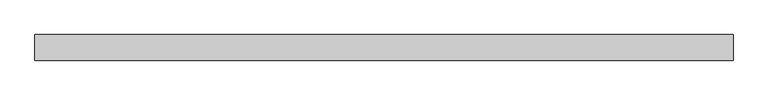
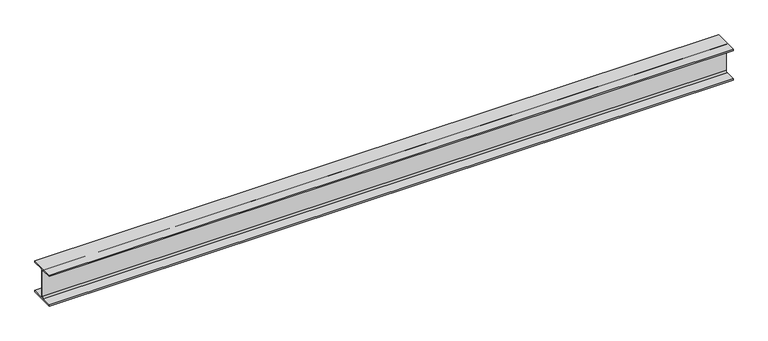
"""IFC4 building model written with IfcOpenShell, lengths in millimetres: beam geometry, 0912_Steel Framing_H-KSD3502 : H_SB_ASB_H-390x300x10x16."""

import ifcopenshell
import ifcopenshell.guid

model = None  # the IFC model being written
_history = None  # IfcOwnerHistory: only IFC2X3 demands one
_inside = {}  # id of a spatial element -> (the spatial element, [elements in it])
_under = {}  # id of a project, library or spatial element -> (it, [spatial elements below it])
_declared = {}  # id of a project -> (the project, [libraries it declares])
_typed = {}  # id of a type object -> (the type object, [elements of that type])
_made_of = {}  # id of a material, layer set ... -> (it, [elements and type objects made of it])


def new_model(schema):
    """Start an empty IFC model of exactly this schema.

    Asked for "IFC4X3", IfcOpenShell would pick the latest addendum, in which some entities
    have other attributes; the version numbers below select the first issue.
    IFC2X3 requires an IfcOwnerHistory on every rooted entity: one is made here for all.
    """
    global model, _history
    if schema == "IFC4X3":
        model = ifcopenshell.file(schema_version=(4, 3, 0, 0))
    else:
        model = ifcopenshell.file(schema=schema)
    _inside.clear()
    _under.clear()
    _declared.clear()
    _typed.clear()
    _made_of.clear()
    _history = None
    if model.schema == "IFC2X3":
        org = make("IfcOrganization", Name="unknown")
        user = make(
            "IfcPersonAndOrganization",
            ThePerson=make("IfcPerson", FamilyName="unknown"),
            TheOrganization=org,
        )
        app = make(
            "IfcApplication",
            ApplicationDeveloper=org,
            Version="unknown",
            ApplicationFullName="unknown",
            ApplicationIdentifier="unknown",
        )
        _history = make(
            "IfcOwnerHistory",
            OwningUser=user,
            OwningApplication=app,
            ChangeAction="ADDED",
            CreationDate=0,
        )
    return model


def make(cls, **values):
    """One entity of the class cls with the attributes given. An attribute that is None is left unset."""
    return model.create_entity(
        cls, **{name: value for name, value in values.items() if value is not None}
    )


def rooted(cls, **values):
    """An entity with a GlobalId (a new one), such as an element, a storey or a relation."""
    return make(cls, GlobalId=ifcopenshell.guid.new(), OwnerHistory=_history, **values)


def si_unit(unit_type, name, prefix=None):
    """IfcSIUnit, for example si_unit("LENGTHUNIT", "METRE", prefix="MILLI")."""
    return make("IfcSIUnit", UnitType=unit_type, Prefix=prefix, Name=name)


def assignment(units):
    """IfcUnitAssignment: the units of a project."""
    return None if units is None else make("IfcUnitAssignment", Units=units)


def point(xyz):
    """IfcCartesianPoint."""
    return None if xyz is None else make("IfcCartesianPoint", Coordinates=xyz)


def direction(xyz):
    """IfcDirection."""
    return None if xyz is None else make("IfcDirection", DirectionRatios=xyz)


def frame(location, z_axis=None, x_axis=None):
    """IfcAxis2Placement3D, a coordinate frame: its origin and axes. An axis left out is left unset."""
    return make(
        "IfcAxis2Placement3D",
        Location=point(location),
        Axis=direction(z_axis),
        RefDirection=direction(x_axis),
    )


def frame_2d(location, x_axis=None):
    """IfcAxis2Placement2D, a coordinate frame in the plane: its origin and x axis."""
    return make(
        "IfcAxis2Placement2D", Location=point(location), RefDirection=direction(x_axis)
    )


def origin():
    """The frame at (0, 0, 0) with its axes left unset."""
    return frame((0.0, 0.0, 0.0))


def place(relative_to, where):
    """IfcLocalPlacement: puts the frame where relative to a parent placement (None: the world)."""
    return make(
        "IfcLocalPlacement", PlacementRelTo=relative_to, RelativePlacement=where
    )


def context(
    kind, dimensions, precision=None, world=None, true_north=None, identifier=None
):
    """IfcGeometricRepresentationContext, for example the 3D "Model" context."""
    return make(
        "IfcGeometricRepresentationContext",
        ContextIdentifier=identifier,
        ContextType=kind,
        CoordinateSpaceDimension=dimensions,
        Precision=precision,
        WorldCoordinateSystem=world,
        TrueNorth=true_north,
    )


def project(units=None, contexts=None):
    """IfcProject with its units and contexts."""
    return rooted(
        "IfcProject",
        Name="project",
        RepresentationContexts=contexts,
        UnitsInContext=assignment(units),
    )


def spatial(cls, under=None, at=None, **own):
    """A site, building, storey or space (cls), placed at a placement, below another one or the project."""
    s = rooted(cls, ObjectPlacement=at, **own)
    if under is not None:
        _under.setdefault(under.id(), (under, []))[1].append(s)
    return s


def polyline(points):
    """IfcPolyline through the points."""
    return make("IfcPolyline", Points=[point(p) for p in points])


def circle_curve(where, radius):
    """IfcCircle in the frame where."""
    return make("IfcCircle", Position=where, Radius=radius)


def trimmed(basis, trim1, trim2, sense, master):
    """IfcTrimmedCurve: the piece of a basis curve between two trims."""
    return make(
        "IfcTrimmedCurve",
        BasisCurve=basis,
        Trim1=trim1,
        Trim2=trim2,
        SenseAgreement=sense,
        MasterRepresentation=master,
    )


def segment(curve, same_sense, transition):
    """IfcCompositeCurveSegment."""
    return make(
        "IfcCompositeCurveSegment",
        Transition=transition,
        SameSense=same_sense,
        ParentCurve=curve,
    )


def composite_curve(segments, self_intersect=None):
    """IfcCompositeCurve: segments joined end to end."""
    return make("IfcCompositeCurve", Segments=segments, SelfIntersect=self_intersect)


def outline(outer, holes=None, kind="AREA"):
    """IfcArbitraryClosedProfileDef: a profile drawn as a closed curve; with holes, ...WithVoids."""
    if holes is None:
        return make("IfcArbitraryClosedProfileDef", ProfileType=kind, OuterCurve=outer)
    return make(
        "IfcArbitraryProfileDefWithVoids",
        ProfileType=kind,
        OuterCurve=outer,
        InnerCurves=holes,
    )


def extrude(swept, where, along, depth):
    """IfcExtrudedAreaSolid: the profile swept, set in the frame where, extruded along a direction by depth."""
    return make(
        "IfcExtrudedAreaSolid",
        SweptArea=swept,
        Position=where,
        ExtrudedDirection=direction(along),
        Depth=depth,
    )


def shape(context_of_items, identifier, shape_type, items):
    """IfcShapeRepresentation: the items that make up one representation, for example the "Body"."""
    return make(
        "IfcShapeRepresentation",
        ContextOfItems=context_of_items,
        RepresentationIdentifier=identifier,
        RepresentationType=shape_type,
        Items=items,
    )


def source(mapping_origin, context_of_items, identifier, shape_type, items):
    """IfcRepresentationMap: a shape defined once, which mapped items show again and again."""
    return make(
        "IfcRepresentationMap",
        MappingOrigin=mapping_origin,
        MappedRepresentation=shape(context_of_items, identifier, shape_type, items),
    )


def transform(
    local_origin,
    x_axis=None,
    y_axis=None,
    z_axis=None,
    scale=None,
    scale2=None,
    scale3=None,
    uniform=True,
):
    """IfcCartesianTransformationOperator3D, or its non-uniform kind. x_axis, y_axis, z_axis: its Axis1, 2, 3."""
    if uniform:
        return make(
            "IfcCartesianTransformationOperator3D",
            Axis1=direction(x_axis),
            Axis2=direction(y_axis),
            LocalOrigin=point(local_origin),
            Scale=scale,
            Axis3=direction(z_axis),
        )
    return make(
        "IfcCartesianTransformationOperator3DnonUniform",
        Axis1=direction(x_axis),
        Axis2=direction(y_axis),
        LocalOrigin=point(local_origin),
        Scale=scale,
        Axis3=direction(z_axis),
        Scale2=scale2,
        Scale3=scale3,
    )


def mapped(mapping_source, mapping_target):
    """IfcMappedItem: shows the shape of a source again, moved by a transform."""
    return make(
        "IfcMappedItem", MappingSource=mapping_source, MappingTarget=mapping_target
    )


def made_of(thing, what):
    """Note that an element or type object is made of a material, layer set ...; save() writes the relation."""
    if what is not None:
        _made_of.setdefault(what.id(), (what, []))[1].append(thing)
    return thing


def element(
    cls,
    number,
    at=None,
    inside=None,
    cuts=None,
    type_object=None,
    material=None,
    context=None,
    identifier="Body",
    shape_type=None,
    held_by="IfcProductDefinitionShape",
    body=None,
    shapes=None,
    **own,
):
    """One element of the class cls, such as IfcWall. Its Tag is "e" and its number.

    at: its placement. inside: the storey or other place that contains it. cuts: it is an
    opening in that element (IfcRelVoidsElement). A single representation is given by context,
    identifier, shape_type and body (its items); several are given by shapes. held_by: the class
    of the entity that holds the representations. save() writes the other relations.
    """
    e = rooted(cls, Tag="e%d" % number, ObjectPlacement=at, **own)
    if body is not None:
        shapes = [shape(context, identifier, shape_type, body)]
    if shapes is not None:
        e.Representation = make(held_by, Representations=shapes)
    if inside is not None:
        _inside.setdefault(inside.id(), (inside, []))[1].append(e)
    if cuts is not None:
        rooted(
            "IfcRelVoidsElement", RelatingBuildingElement=cuts, RelatedOpeningElement=e
        )
    if type_object is not None:
        _typed.setdefault(type_object.id(), (type_object, []))[1].append(e)
    return made_of(e, material)


def aggregate(whole, parts):
    """IfcRelAggregates: a whole, such as a stair, and the parts it consists of."""
    return rooted("IfcRelAggregates", RelatingObject=whole, RelatedObjects=parts)


def save(model, path):
    """Write the relations noted so far, then the file.

    IfcRelAggregates (storeys below a building ...), IfcRelContainedInSpatialStructure (elements
    in a storey), IfcRelDefinesByType, IfcRelAssociatesMaterial and IfcRelDeclares: one each for
    every whole, place, type object, material and project.
    """
    for whole, parts in _under.values():
        aggregate(whole, parts)
    for where, things in _inside.values():
        rooted(
            "IfcRelContainedInSpatialStructure",
            RelatedElements=things,
            RelatingStructure=where,
        )
    for kind, things in _typed.values():
        rooted("IfcRelDefinesByType", RelatedObjects=things, RelatingType=kind)
    for what, things in _made_of.values():
        rooted("IfcRelAssociatesMaterial", RelatedObjects=things, RelatingMaterial=what)
    for by, libraries in _declared.values():
        rooted("IfcRelDeclares", RelatingContext=by, RelatedDefinitions=libraries)
    model.write(path)


def beam_d2c522c6(model_context):
    return source(origin(), model_context, "Body", "SweptSolid", [
        extrude(outline(composite_curve([segment(polyline([(150.0, -179.0), (150.0, -195.0), (-150.0, -195.0), (-150.0, -179.0), (-27.0, -179.0)]), True, "CONTINUOUS"), segment(trimmed(circle_curve(frame_2d((-27.0, -157.0)), 22.0), [point((-27.0, -179.0))], [point((-5.0, -157.0))], True, "CARTESIAN"), True, "CONTINUOUS"), segment(polyline([(-5.0, -157.0), (-5.0, 157.0)]), True, "CONTINUOUS"), segment(trimmed(circle_curve(frame_2d((-27.0, 157.0)), 22.0), [point((-5.0, 157.0))], [point((-27.0, 179.0))], True, "CARTESIAN"), True, "CONTINUOUS"), segment(polyline([(-27.0, 179.0), (-150.0, 179.0), (-150.0, 195.0), (150.0, 195.0), (150.0, 179.0), (27.0, 179.0)]), True, "CONTINUOUS"), segment(trimmed(circle_curve(frame_2d((27.0, 157.0)), 22.0), [point((27.0, 179.0))], [point((5.0, 157.0))], True, "CARTESIAN"), True, "CONTINUOUS"), segment(polyline([(5.0, 157.0), (5.0, -157.0)]), True, "CONTINUOUS"), segment(trimmed(circle_curve(frame_2d((27.0, -157.0)), 22.0), [point((5.0, -157.0))], [point((27.0, -179.0))], True, "CARTESIAN"), True, "CONTINUOUS"), segment(polyline([(27.0, -179.0), (150.0, -179.0)]), True, "CONTINUOUS")], self_intersect=False)), frame((-4087.3, 0.0, 0.0), z_axis=(1.0, 0.0, 0.0), x_axis=(0.0, 1.0, 0.0)), (0.0, 0.0, 1.0), 8174.6),
    ])


if __name__ == "__main__":
    model = new_model("IFC4")
    model_context = context("Model", 3, world=origin())
    ifc_project = project(units=[si_unit("LENGTHUNIT", "METRE", prefix="MILLI")], contexts=[model_context])
    site = spatial("IfcSite", under=ifc_project)
    building = spatial("IfcBuilding", under=site)
    placement = place(None, origin())
    beam_shape = beam_d2c522c6(model_context)
    element("IfcBeam", 1, ObjectType="0912_Steel Framing_H-KSD3502 : H_SB_ASB_H-390x300x10x16", at=placement, inside=building, context=model_context, shape_type="MappedRepresentation", body=[
        mapped(beam_shape, transform((0.0, 0.0, 0.0), x_axis=(1.0, 0.0, 0.0), y_axis=(0.0, 1.0, 0.0), z_axis=(0.0, 0.0, 1.0))),
    ])
    save(model, "model.ifc")

# Revit data of these elements
# Type "0912_Steel Framing_H-KSD3502 : H_SB_ASB_H-390x300x10x16"
#   H_WM Code_1 = "S01AA001-00001 | Main Steel Structure Fabrication Work | Shelter/Building | Heavy Steel - Standard (Weight≥90KG/M) | Material: (   )"
#   H_WM Code_2 = "S03AA027-00001 | Main Steel Structure Erection Work | Shelter/Building | Heavy Steel (Weight≥90KG/M) | Material: (   )"
#   H_WM Code_3 = "S01AA010-00001 | Main Steel Structure Fabrication Work | Shelter/Building | Steel Painting/Coating | for Non-Fireproofed Steel Surface, Surface Preparation, Primer, Second & Final Coat | Material: (   )"
#   H_Q'ty Cal Type Tag = "SB-Q2"
#   Width = 30.0 cm
#   Web Thickness = 1.0 cm
#   Web Fillet = 2.2 cm
#   Warping Constant = 2520000.0 cm⁶
#   W = 0
#   Torsional Moment of Inertia = 94.3867 cm⁴
#   Section Area = 136.0 cm²
#   Plastic Modulus weak axis = 733.0 cm³
#   Plastic Modulus strong axis = 2190.0 cm³
#   Perimeter = 1.92 m²/m
#   Nominal Weight = 107.00 kgf/m
#   Moment of Inertia weak axis = 7210.00 cm⁴
#   Moment of Inertia strong axis = 38700.00 cm⁴
#   Height = 39.0 cm
#   Flange Thickness = 1.6 cm
#   Elastic Modulus weak axis = 481.0 cm³
#   Elastic Modulus strong axis = 1980.0 cm³
#   Centroid Vertical = 19.5 cm
#   Centroid Horizontal = 15.0 cm
#   Ix = 387000000
#   Length [instance default] = 1.5240 m
#   Zx = 2190000
#   b = 0.3000 m
#   h = 0.3900 m
#   r = 0.0220 m
#   s = 0.0100 m
#   t = 0.0160 m
#   A = 0.0136 m²
#   Structural Material [instance default] = Steel, 45-345
#   Assembly Code = ""
# Element 1 (IfcBeam, "0912_Steel Framing_H-KSD3502 : H_SB_ASB_H-390x300x10x16")
#   Structural Material = none
# Materials
#   "Steel, 45-345": class "Metal", colour RGB 189 187 185, transparency 0, Description = "Steel 345 MPa", Cost = 0
